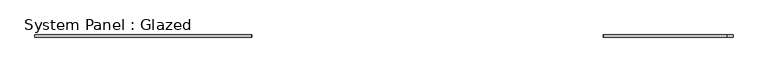
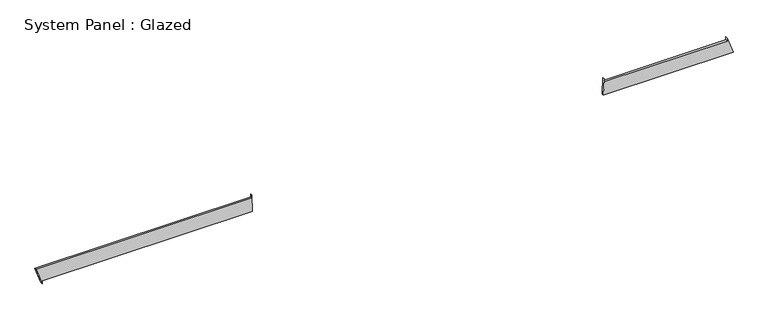
"""IFC4 building model written with IfcOpenShell, lengths in millimetres: plate geometry, System Panel : Glazed."""

from ifc_helpers import new_model, si_unit, frame, origin, place, context, project, spatial, polyline, outline, extrude, source, transform, mapped, element, save


def system_panel_glazed_f0fb4d28(model_context):
    return source(origin(), model_context, "Body", "SweptSolid", [
        extrude(outline(polyline([(0.0, -3957.920533), (35.3553391, -3957.920533), (35.3553391, -1528.3824564), (234.5648417, -1533.0425335), (199.2095027, -1533.041855), (199.1616377, -4027.1611563), (0.0, -3957.920533)])), frame((0.0, -49.5, 0.0), z_axis=(0.0, 1.0, 0.0), x_axis=(0.0, 0.0, 1.0)), (0.0, 0.0, 1.0), 25.0),
        extrude(outline(polyline([(35.3553391, 2529.1821165), (35.3553391, 4027.1611563), (234.6702265, 3958.2886876), (199.3148875, 3958.2893661), (199.2876112, 2536.9935327), (234.6429503, 2536.9928542), (35.3553391, 2529.1821165)])), frame((0.0, -49.5, 0.0), z_axis=(0.0, 1.0, 0.0), x_axis=(0.0, 0.0, 1.0)), (0.0, 0.0, 1.0), 25.0),
    ])


if __name__ == "__main__":
    model = new_model("IFC4")
    model_context = context("Model", 3, world=origin())
    ifc_project = project(units=[si_unit("LENGTHUNIT", "METRE", prefix="MILLI")], contexts=[model_context])
    site = spatial("IfcSite", under=ifc_project)
    building = spatial("IfcBuilding", under=site)
    placement = place(None, origin())
    system_panel_glazed_shape = system_panel_glazed_f0fb4d28(model_context)
    element("IfcPlate", 1, ObjectType="System Panel : Glazed", at=placement, inside=building, context=model_context, shape_type="MappedRepresentation", body=[
        mapped(system_panel_glazed_shape, transform((0.0, 0.0, 0.0), x_axis=(1.0, 0.0, 0.0), y_axis=(0.0, 1.0, 0.0), z_axis=(0.0, 0.0, 1.0))),
    ])
    save(model, "model.ifc")

# Revit data of these elements
# Element 1 (IfcPlate, "System Panel : Glazed")
#   Materials on its faces: "Glass"
# Materials
#   "Glass": class "Glass", colour RGB 218 227 224, transparency 0.85, Description = "Soda Lime Glass", Cost = 0
